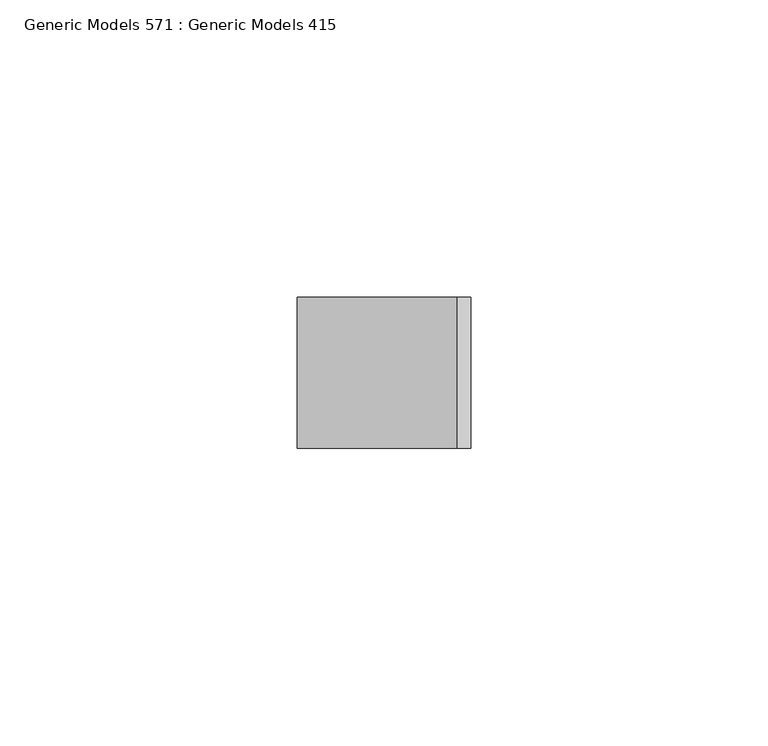
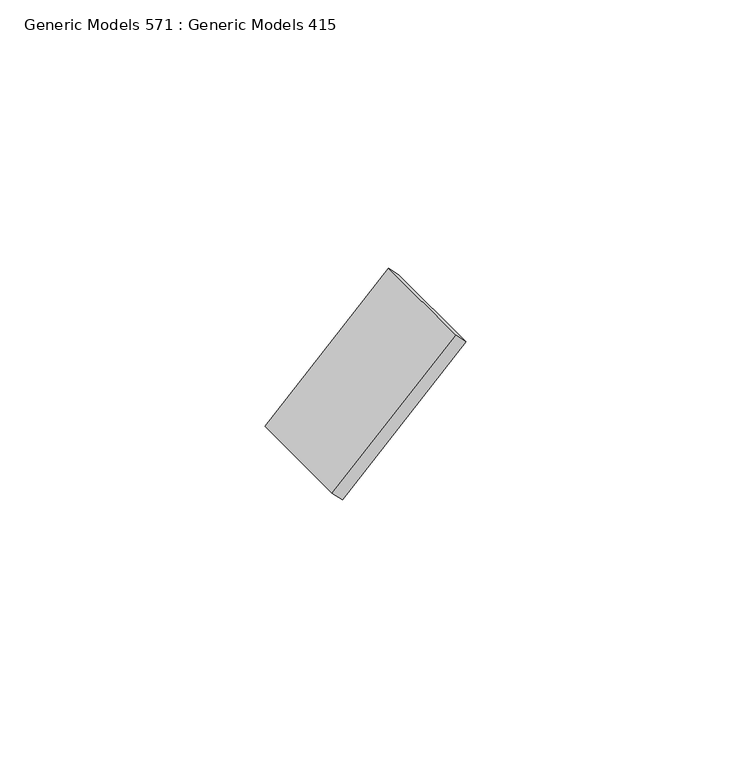
"""IFC4 building model written with IfcOpenShell, lengths in millimetres: proxy geometry, Generic Models 571 : Generic Models 415."""

from ifc_helpers import new_model, si_unit, frame, origin, place, context, project, spatial, polyline, outline, extrude, source, transform, mapped, element, save


def generic_models_571_generic_models_415_bd67c941(model_context):
    return source(origin(), model_context, "Body", "SweptSolid", [
        extrude(outline(polyline([(0.0, -3.175), (0.0, 0.0), (25.4, 0.0), (25.4, -3.175), (0.0, -3.175)])), frame((7848.0411784, 4501.3863946, 124051.3849742), z_axis=(0.7071067811867181, 0.0, 0.707106781186377), x_axis=(0.0, -1.0, 0.0)), (0.0, 0.0, 1.0), 38.1),
    ])


if __name__ == "__main__":
    model = new_model("IFC4")
    model_context = context("Model", 3, world=origin())
    ifc_project = project(units=[si_unit("LENGTHUNIT", "METRE", prefix="MILLI")], contexts=[model_context])
    site = spatial("IfcSite", under=ifc_project)
    building = spatial("IfcBuilding", under=site)
    placement = place(None, origin())
    generic_models_571_generic_models_415_shape = generic_models_571_generic_models_415_bd67c941(model_context)
    element("IfcBuildingElementProxy", 1, Name="Generic Models 571 : Generic Models 415", ObjectType="Generic Models 571 : Generic Models 415", at=placement, inside=building, context=model_context, shape_type="MappedRepresentation", body=[
        mapped(generic_models_571_generic_models_415_shape, transform((0.0, 0.0, 0.0), x_axis=(1.0, 0.0, 0.0), y_axis=(0.0, 1.0, 0.0), z_axis=(0.0, 0.0, 1.0))),
    ])
    save(model, "model.ifc")

# Revit data of these elements
# Element 1 (IfcBuildingElementProxy, "Generic Models 571 : Generic Models 415")
#   Materials on its faces: "_WELDED STEEL TABS FOR LOUVER ATTACHMENT"
# Materials
#   "_WELDED STEEL TABS FOR LOUVER ATTACHMENT": class "Metal", colour RGB 199 199 199, transparency 0, Description = "Structural steel 50ksi", Cost = 0
